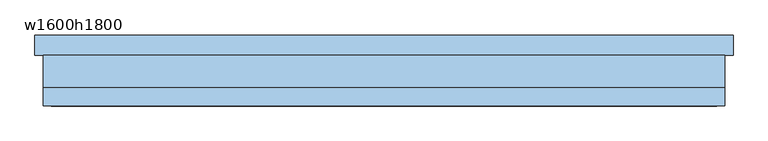
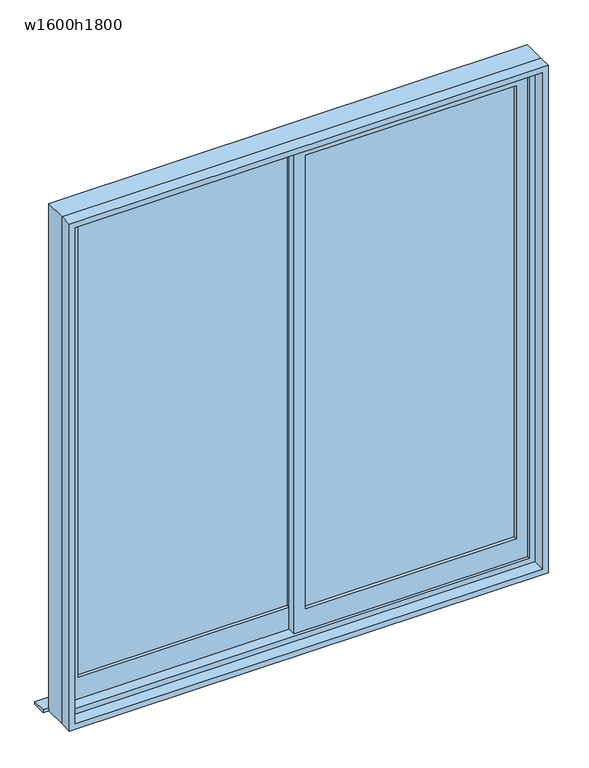
"""IFC4 building model written with IfcOpenShell, lengths in millimetres: window geometry, 引違い掃出窓_2枚 : w1600h1800."""

from ifc_helpers import new_model, si_unit, frame, origin, place, context, project, spatial, polyline, outline, extrude, source, transform, mapped, element, save


def w1600h1800_8e15063a(model_context):
    return source(origin(), model_context, "Body", "SweptSolid", [
        extrude(outline(polyline([(-20.0, 12.5), (-760.0, 12.5), (-760.0, 17.5), (-20.0, 17.5), (-20.0, 12.5)])), frame((0.0, 0.0, 280.0), z_axis=(0.0, 0.0, 1.0), x_axis=(1.0, 0.0, 0.0)), (0.0, 0.0, 1.0), 1680.0),
        extrude(outline(polyline([(760.0, -17.5), (20.0, -17.5), (20.0, -12.5), (760.0, -12.5), (760.0, -17.5)])), frame((0.0, 0.0, 280.0), z_axis=(0.0, 0.0, 1.0), x_axis=(1.0, 0.0, 0.0)), (0.0, 0.0, 1.0), 1680.0),
        extrude(outline(polyline([(2000.0, -20.0), (200.0, -20.0), (200.0, 800.0), (2000.0, 800.0), (2000.0, -20.0)]), holes=[polyline([(280.0, 760.0), (280.0, 20.0), (1960.0, 20.0), (1960.0, 760.0), (280.0, 760.0)])]), frame((0.0, -30.0, 0.0), z_axis=(0.0, 1.0, 0.0), x_axis=(0.0, 0.0, 1.0)), (0.0, 0.0, 1.0), 30.0),
        extrude(outline(polyline([(2000.0, -800.0), (200.0, -800.0), (200.0, 20.0), (2000.0, 20.0), (2000.0, -800.0)]), holes=[polyline([(280.0, -20.0), (280.0, -760.0), (1960.0, -760.0), (1960.0, -20.0), (280.0, -20.0)])]), frame((0.0, 0.0, 0.0), z_axis=(0.0, 1.0, 0.0), x_axis=(0.0, 0.0, 1.0)), (0.0, 0.0, 1.0), 30.0),
        extrude(outline(polyline([(860.0, 90.0), (860.0, 40.0), (-860.0, 40.0), (-860.0, 90.0), (860.0, 90.0)])), frame((0.0, 0.0, 160.0), z_axis=(0.0, 0.0, 1.0), x_axis=(1.0, 0.0, 0.0)), (0.0, 0.0, 1.0), 10.0),
        extrude(outline(polyline([(2040.0, 840.0), (2040.0, -840.0), (160.0, -840.0), (160.0, 840.0), (2040.0, 840.0)]), holes=[polyline([(180.0, -820.0), (2020.0, -820.0), (2020.0, 820.0), (180.0, 820.0), (180.0, -820.0)])]), frame((0.0, -85.0, 0.0), z_axis=(0.0, 1.0, 0.0), x_axis=(0.0, 0.0, 1.0)), (0.0, 0.0, 1.0), 45.0),
        extrude(outline(polyline([(2040.0, -840.0), (160.0, -840.0), (160.0, 840.0), (2040.0, 840.0), (2040.0, -840.0)]), holes=[polyline([(2000.0, 800.0), (200.0, 800.0), (200.0, -800.0), (2000.0, -800.0), (2000.0, 800.0)])]), frame((0.0, -40.0, 0.0), z_axis=(0.0, 1.0, 0.0), x_axis=(0.0, 0.0, 1.0)), (0.0, 0.0, 1.0), 80.0),
    ])


if __name__ == "__main__":
    model = new_model("IFC4")
    model_context = context("Model", 3, world=origin())
    ifc_project = project(units=[si_unit("LENGTHUNIT", "METRE", prefix="MILLI")], contexts=[model_context])
    site = spatial("IfcSite", under=ifc_project)
    building = spatial("IfcBuilding", under=site)
    placement = place(None, origin())
    w1600h1800_shape = w1600h1800_8e15063a(model_context)
    element("IfcWindow", 1, ObjectType="引違い掃出窓_2枚 : w1600h1800", at=placement, inside=building, context=model_context, shape_type="MappedRepresentation", body=[
        mapped(w1600h1800_shape, transform((0.0, 0.0, 0.0), x_axis=(1.0, 0.0, 0.0), y_axis=(0.0, 1.0, 0.0), z_axis=(0.0, 0.0, 1.0))),
    ])
    save(model, "model.ifc")

# Revit data of these elements
# Type "引違い掃出窓_2枚 : w1600h1800"
#   Construction Type Id = "GSP4R"
#   Analytic Construction = "1/8 インチ ピルキントン一重ガラス"
#   Type Mark = "67"
#   Operation = "ダブル パネル縦"
#   Keynote = "08520.R1"
#   Visual Light Transmittance = 0.9
#   Solar Heat Gain Coefficient = 0.86
#   Heat Transfer Coefficient (U) = 6.7069 W/(m²·K)
#   Height = 1800 mm
#   既定の腰高 = 200 mm
#   Width = 1600 mm
#   額縁見附 = 20 mm
#   額縁ちり = 10 mm
#   サッシ見附 = 40 mm
#   サッシの幅 = 80 mm
#   サッシ額縁 [instance default] = none
#   サッシ本体 [instance default] = none
#   サッシガラス [instance default] = ガラス - 透明
#   Manufacturer = ""
#   Wall Closure = (empty or 0)
#   Model = ""
#   Type Comments = ""
#   Assembly Code = ""
# Element 1 (IfcWindow, "引違い掃出窓_2枚 : w1600h1800")
#   Materials on its faces: "ガラス - 透明"
# Materials
#   "ガラス - 透明": class "ガラス", colour RGB 0 128 192, transparency 0.9, Cost = 0
